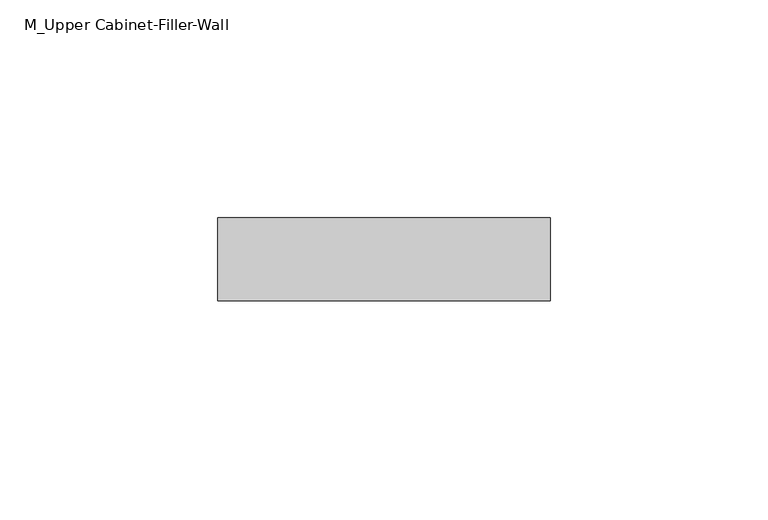
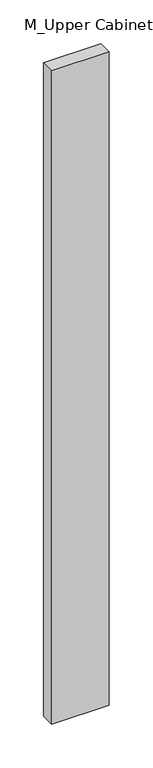
"""IFC4 building model written with IfcOpenShell, lengths in millimetres: furniture geometry, M_Upper Cabinet-Filler-Wall : Fverticle1 3."""

import ifcopenshell
import ifcopenshell.guid

model = None  # the IFC model being written
_history = None  # IfcOwnerHistory: only IFC2X3 demands one
_inside = {}  # id of a spatial element -> (the spatial element, [elements in it])
_under = {}  # id of a project, library or spatial element -> (it, [spatial elements below it])
_declared = {}  # id of a project -> (the project, [libraries it declares])
_typed = {}  # id of a type object -> (the type object, [elements of that type])
_made_of = {}  # id of a material, layer set ... -> (it, [elements and type objects made of it])


def new_model(schema):
    """Start an empty IFC model of exactly this schema.

    Asked for "IFC4X3", IfcOpenShell would pick the latest addendum, in which some entities
    have other attributes; the version numbers below select the first issue.
    IFC2X3 requires an IfcOwnerHistory on every rooted entity: one is made here for all.
    """
    global model, _history
    if schema == "IFC4X3":
        model = ifcopenshell.file(schema_version=(4, 3, 0, 0))
    else:
        model = ifcopenshell.file(schema=schema)
    _inside.clear()
    _under.clear()
    _declared.clear()
    _typed.clear()
    _made_of.clear()
    _history = None
    if model.schema == "IFC2X3":
        org = make("IfcOrganization", Name="unknown")
        user = make(
            "IfcPersonAndOrganization",
            ThePerson=make("IfcPerson", FamilyName="unknown"),
            TheOrganization=org,
        )
        app = make(
            "IfcApplication",
            ApplicationDeveloper=org,
            Version="unknown",
            ApplicationFullName="unknown",
            ApplicationIdentifier="unknown",
        )
        _history = make(
            "IfcOwnerHistory",
            OwningUser=user,
            OwningApplication=app,
            ChangeAction="ADDED",
            CreationDate=0,
        )
    return model


def make(cls, **values):
    """One entity of the class cls with the attributes given. An attribute that is None is left unset."""
    return model.create_entity(
        cls, **{name: value for name, value in values.items() if value is not None}
    )


def rooted(cls, **values):
    """An entity with a GlobalId (a new one), such as an element, a storey or a relation."""
    return make(cls, GlobalId=ifcopenshell.guid.new(), OwnerHistory=_history, **values)


def si_unit(unit_type, name, prefix=None):
    """IfcSIUnit, for example si_unit("LENGTHUNIT", "METRE", prefix="MILLI")."""
    return make("IfcSIUnit", UnitType=unit_type, Prefix=prefix, Name=name)


def assignment(units):
    """IfcUnitAssignment: the units of a project."""
    return None if units is None else make("IfcUnitAssignment", Units=units)


def point(xyz):
    """IfcCartesianPoint."""
    return None if xyz is None else make("IfcCartesianPoint", Coordinates=xyz)


def direction(xyz):
    """IfcDirection."""
    return None if xyz is None else make("IfcDirection", DirectionRatios=xyz)


def frame(location, z_axis=None, x_axis=None):
    """IfcAxis2Placement3D, a coordinate frame: its origin and axes. An axis left out is left unset."""
    return make(
        "IfcAxis2Placement3D",
        Location=point(location),
        Axis=direction(z_axis),
        RefDirection=direction(x_axis),
    )


def origin():
    """The frame at (0, 0, 0) with its axes left unset."""
    return frame((0.0, 0.0, 0.0))


def place(relative_to, where):
    """IfcLocalPlacement: puts the frame where relative to a parent placement (None: the world)."""
    return make(
        "IfcLocalPlacement", PlacementRelTo=relative_to, RelativePlacement=where
    )


def context(
    kind, dimensions, precision=None, world=None, true_north=None, identifier=None
):
    """IfcGeometricRepresentationContext, for example the 3D "Model" context."""
    return make(
        "IfcGeometricRepresentationContext",
        ContextIdentifier=identifier,
        ContextType=kind,
        CoordinateSpaceDimension=dimensions,
        Precision=precision,
        WorldCoordinateSystem=world,
        TrueNorth=true_north,
    )


def project(units=None, contexts=None):
    """IfcProject with its units and contexts."""
    return rooted(
        "IfcProject",
        Name="project",
        RepresentationContexts=contexts,
        UnitsInContext=assignment(units),
    )


def spatial(cls, under=None, at=None, **own):
    """A site, building, storey or space (cls), placed at a placement, below another one or the project."""
    s = rooted(cls, ObjectPlacement=at, **own)
    if under is not None:
        _under.setdefault(under.id(), (under, []))[1].append(s)
    return s


def polyline(points):
    """IfcPolyline through the points."""
    return make("IfcPolyline", Points=[point(p) for p in points])


def outline(outer, holes=None, kind="AREA"):
    """IfcArbitraryClosedProfileDef: a profile drawn as a closed curve; with holes, ...WithVoids."""
    if holes is None:
        return make("IfcArbitraryClosedProfileDef", ProfileType=kind, OuterCurve=outer)
    return make(
        "IfcArbitraryProfileDefWithVoids",
        ProfileType=kind,
        OuterCurve=outer,
        InnerCurves=holes,
    )


def extrude(swept, where, along, depth):
    """IfcExtrudedAreaSolid: the profile swept, set in the frame where, extruded along a direction by depth."""
    return make(
        "IfcExtrudedAreaSolid",
        SweptArea=swept,
        Position=where,
        ExtrudedDirection=direction(along),
        Depth=depth,
    )


def shape(context_of_items, identifier, shape_type, items):
    """IfcShapeRepresentation: the items that make up one representation, for example the "Body"."""
    return make(
        "IfcShapeRepresentation",
        ContextOfItems=context_of_items,
        RepresentationIdentifier=identifier,
        RepresentationType=shape_type,
        Items=items,
    )


def source(mapping_origin, context_of_items, identifier, shape_type, items):
    """IfcRepresentationMap: a shape defined once, which mapped items show again and again."""
    return make(
        "IfcRepresentationMap",
        MappingOrigin=mapping_origin,
        MappedRepresentation=shape(context_of_items, identifier, shape_type, items),
    )


def transform(
    local_origin,
    x_axis=None,
    y_axis=None,
    z_axis=None,
    scale=None,
    scale2=None,
    scale3=None,
    uniform=True,
):
    """IfcCartesianTransformationOperator3D, or its non-uniform kind. x_axis, y_axis, z_axis: its Axis1, 2, 3."""
    if uniform:
        return make(
            "IfcCartesianTransformationOperator3D",
            Axis1=direction(x_axis),
            Axis2=direction(y_axis),
            LocalOrigin=point(local_origin),
            Scale=scale,
            Axis3=direction(z_axis),
        )
    return make(
        "IfcCartesianTransformationOperator3DnonUniform",
        Axis1=direction(x_axis),
        Axis2=direction(y_axis),
        LocalOrigin=point(local_origin),
        Scale=scale,
        Axis3=direction(z_axis),
        Scale2=scale2,
        Scale3=scale3,
    )


def mapped(mapping_source, mapping_target):
    """IfcMappedItem: shows the shape of a source again, moved by a transform."""
    return make(
        "IfcMappedItem", MappingSource=mapping_source, MappingTarget=mapping_target
    )


def made_of(thing, what):
    """Note that an element or type object is made of a material, layer set ...; save() writes the relation."""
    if what is not None:
        _made_of.setdefault(what.id(), (what, []))[1].append(thing)
    return thing


def element(
    cls,
    number,
    at=None,
    inside=None,
    cuts=None,
    type_object=None,
    material=None,
    context=None,
    identifier="Body",
    shape_type=None,
    held_by="IfcProductDefinitionShape",
    body=None,
    shapes=None,
    **own,
):
    """One element of the class cls, such as IfcWall. Its Tag is "e" and its number.

    at: its placement. inside: the storey or other place that contains it. cuts: it is an
    opening in that element (IfcRelVoidsElement). A single representation is given by context,
    identifier, shape_type and body (its items); several are given by shapes. held_by: the class
    of the entity that holds the representations. save() writes the other relations.
    """
    e = rooted(cls, Tag="e%d" % number, ObjectPlacement=at, **own)
    if body is not None:
        shapes = [shape(context, identifier, shape_type, body)]
    if shapes is not None:
        e.Representation = make(held_by, Representations=shapes)
    if inside is not None:
        _inside.setdefault(inside.id(), (inside, []))[1].append(e)
    if cuts is not None:
        rooted(
            "IfcRelVoidsElement", RelatingBuildingElement=cuts, RelatedOpeningElement=e
        )
    if type_object is not None:
        _typed.setdefault(type_object.id(), (type_object, []))[1].append(e)
    return made_of(e, material)


def aggregate(whole, parts):
    """IfcRelAggregates: a whole, such as a stair, and the parts it consists of."""
    return rooted("IfcRelAggregates", RelatingObject=whole, RelatedObjects=parts)


def save(model, path):
    """Write the relations noted so far, then the file.

    IfcRelAggregates (storeys below a building ...), IfcRelContainedInSpatialStructure (elements
    in a storey), IfcRelDefinesByType, IfcRelAssociatesMaterial and IfcRelDeclares: one each for
    every whole, place, type object, material and project.
    """
    for whole, parts in _under.values():
        aggregate(whole, parts)
    for where, things in _inside.values():
        rooted(
            "IfcRelContainedInSpatialStructure",
            RelatedElements=things,
            RelatingStructure=where,
        )
    for kind, things in _typed.values():
        rooted("IfcRelDefinesByType", RelatedObjects=things, RelatingType=kind)
    for what, things in _made_of.values():
        rooted("IfcRelAssociatesMaterial", RelatedObjects=things, RelatingMaterial=what)
    for by, libraries in _declared.values():
        rooted("IfcRelDeclares", RelatingContext=by, RelatedDefinitions=libraries)
    model.write(path)


def m_upper_cabinet_filler_wall_177953ad(model_context):
    return source(origin(), model_context, "Body", "SweptSolid", [
        extrude(outline(polyline([(-8.3288372, 38.1), (-8.3288372, 57.15), (67.8711628, 57.15), (67.8711628, 38.1), (-8.3288372, 38.1)])), frame((0.0, 0.0, 1085.6), z_axis=(0.0, 0.0, 1.0), x_axis=(1.0, 0.0, 0.0)), (0.0, 0.0, 1.0), 914.4),
    ])


if __name__ == "__main__":
    model = new_model("IFC4")
    model_context = context("Model", 3, world=origin())
    ifc_project = project(units=[si_unit("LENGTHUNIT", "METRE", prefix="MILLI")], contexts=[model_context])
    site = spatial("IfcSite", under=ifc_project)
    building = spatial("IfcBuilding", under=site)
    placement = place(None, origin())
    m_upper_cabinet_filler_wall_shape = m_upper_cabinet_filler_wall_177953ad(model_context)
    element("IfcFurniture", 1, ObjectType="M_Upper Cabinet-Filler-Wall : Fverticle1 3", at=placement, inside=building, context=model_context, shape_type="MappedRepresentation", body=[
        mapped(m_upper_cabinet_filler_wall_shape, transform((0.0, 0.0, 0.0), x_axis=(1.0, 0.0, 0.0), y_axis=(0.0, 1.0, 0.0), z_axis=(0.0, 0.0, 1.0))),
    ])
    save(model, "model.ifc")

# Revit data of these elements
# Type "M_Upper Cabinet-Filler-Wall : Fverticle1 3"
#   Depth = 0' - 1"
#   Height = 3' - 0"
#   Top Of Cabinet = 6' - 6.74016"
#   Width = 0' - 3"
#   Cabinet Material = none
#   Default Elevation = 0
# Element 1 (IfcFurniture, "M_Upper Cabinet-Filler-Wall : Fverticle1 3")
#   Materials on its faces: "Cabinets"
# Materials
#   "Cabinets": class "Miscellaneous", colour RGB 249 249 249, transparency 0
